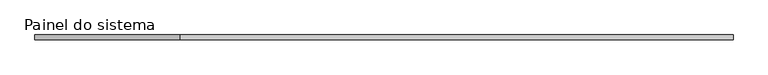
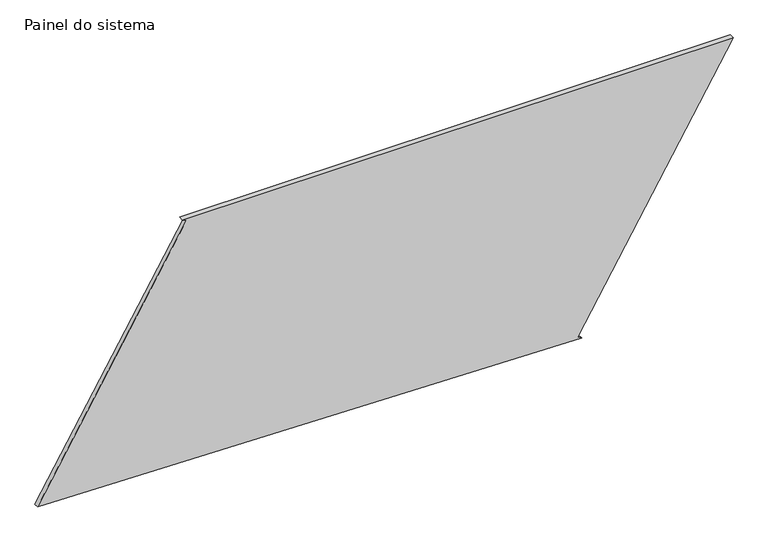
"""IFC4 building model written with IfcOpenShell, lengths in millimetres: plate geometry, Painel do sistema : Envidraçado."""

from ifc_helpers import new_model, si_unit, frame, origin, place, context, project, spatial, polyline, outline, extrude, source, transform, mapped, element, save


def painel_do_sistema_b428a5c0(model_context):
    return source(origin(), model_context, "Body", "SweptSolid", [
        extrude(outline(polyline([(0.0, 1054.6268356), (12.7505939, 1033.1228277), (1423.5378573, 1869.6355216), (1423.5378573, -1092.1715924), (1410.7872633, -1070.6675845), (63.3196186, -1869.6355216), (0.0, 1054.6268356)])), frame((0.0, 24.5, 0.0), z_axis=(0.0, 1.0, 0.0), x_axis=(0.0, 0.0, 1.0)), (0.0, 0.0, 1.0), 25.0),
    ])


if __name__ == "__main__":
    model = new_model("IFC4")
    model_context = context("Model", 3, world=origin())
    ifc_project = project(units=[si_unit("LENGTHUNIT", "METRE", prefix="MILLI")], contexts=[model_context])
    site = spatial("IfcSite", under=ifc_project)
    building = spatial("IfcBuilding", under=site)
    placement = place(None, origin())
    painel_do_sistema_shape = painel_do_sistema_b428a5c0(model_context)
    element("IfcPlate", 1, ObjectType="Painel do sistema : Envidraçado", at=placement, inside=building, context=model_context, shape_type="MappedRepresentation", body=[
        mapped(painel_do_sistema_shape, transform((0.0, 0.0, 0.0), x_axis=(1.0, 0.0, 0.0), y_axis=(0.0, 1.0, 0.0), z_axis=(0.0, 0.0, 1.0))),
    ])
    save(model, "model.ifc")

# Revit data of these elements
# Type "Painel do sistema : Envidraçado"
#   Construction Type Id = "GSP4R"
#   Analytic Construction = "Vidraça única Pilkington 1/8 pol"
#   Visual Light Transmittance = 0.9
#   Solar Heat Gain Coefficient = 0.86
#   Heat Transfer Coefficient (U) = 6.7069 W/(m²·K)
# Element 1 (IfcPlate, "Painel do sistema : Envidraçado")
#   Materials on its faces: "Vidro"
# Materials
#   "Vidro": class "Vidro", colour RGB 0 128 192, transparency 0.9, Description = "Vidro de sílica", Cost = 0
